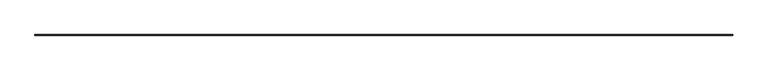
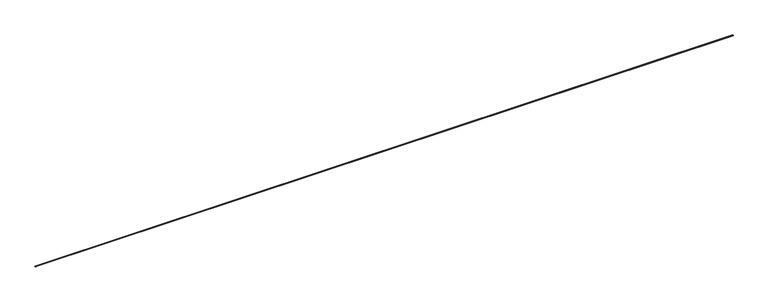
"""IFC4 building model written with IfcOpenShell, lengths in millimetres: proxy geometry, Inner panel:Inner panel:1:Inner panel:1 : Inner panel:Inner panel:300324:2:Inner panel:1:Inner panel:1 : Inner panel:Inner panel:300324:2 : Inner panel:Inner panel:1:Inner panel:1 : Inner panel:Inner panel:300324:300043:43 : Inner panel:Inner panel:1:Inner panel:1 : Inner panel:Inner panel:300324:2:Inner panel:1:Inner panel:1 : Inner panel:Inner panel:300324:2 : Inner panel:Inner panel:1:Inner panel:1 : Inner panel:Inner panel:300324:300043:308120."""

from ifc_helpers import new_model, si_unit, frame, origin, place, context, project, spatial, polyline, outline, extrude, source, transform, mapped, element, save


def generic_models_34035f40(model_context):
    return source(origin(), model_context, "Body", "SweptSolid", [
        extrude(outline(polyline([(-578217.5686142, 3944.3954083), (-578219.0886494, 3980.8762546), (-578261.9668057, 3979.0896648), (-578260.4467705, 3942.6088184), (-578277.1211775, 3941.9140515), (-578277.278418, 3945.6878244), (-578275.6895406, 3945.6878244), (-578275.6011422, 3943.5662637), (-578262.0989827, 3944.1288537), (-578263.619018, 3980.6097), (-578217.5686142, 3982.5284669), (-578216.0485789, 3946.0476205), (-578202.5464194, 3946.6102105), (-578202.6375715, 3948.7978597), (-578201.048694, 3948.7978597), (-578200.8942072, 3945.0901752), (-578217.5686142, 3944.3954083)])), frame((579104.5117239, 0.0, 0.0), z_axis=(1.0, 0.0, 0.0), x_axis=(0.0, 1.0, 0.0)), (0.0, 0.0, 1.0), 88442.8),
    ])


if __name__ == "__main__":
    model = new_model("IFC4")
    model_context = context("Model", 3, world=origin())
    ifc_project = project(units=[si_unit("LENGTHUNIT", "METRE", prefix="MILLI")], contexts=[model_context])
    site = spatial("IfcSite", under=ifc_project)
    building = spatial("IfcBuilding", under=site)
    placement = place(None, origin())
    generic_models_shape = generic_models_34035f40(model_context)
    element("IfcBuildingElementProxy", 1, Name="Inner panel:Inner panel:1:Inner panel:1 : Inner panel:Inner panel:300324:2:Inner panel:1:Inner panel:1 : Inner panel:Inner panel:300324:2 : Inner panel:Inner panel:1:Inner panel:1 : Inner panel:Inner panel:300324:300043:43 : Inner panel:Inner panel:1:Inner panel:1 : Inner panel:Inner panel:300324:2:Inner panel:1:Inner panel:1 : Inner panel:Inner panel:300324:2 : Inner panel:Inner panel:1:Inner panel:1 : Inner panel:Inner panel:300324:300043:308120", ObjectType="Inner panel:Inner panel:1:Inner panel:1 : Inner panel:Inner panel:300324:2:Inner panel:1:Inner panel:1 : Inner panel:Inner panel:300324:2 : Inner panel:Inner panel:1:Inner panel:1 : Inner panel:Inner panel:300324:300043:43 : Inner panel:Inner panel:1:Inner panel:1 : Inner panel:Inner panel:300324:2:Inner panel:1:Inner panel:1 : Inner panel:Inner panel:300324:2 : Inner panel:Inner panel:1:Inner panel:1 : Inner panel:Inner panel:300324:300043:308120", at=placement, inside=building, context=model_context, shape_type="MappedRepresentation", body=[
        mapped(generic_models_shape, transform((0.0, 0.0, 0.0), x_axis=(1.0, 0.0, 0.0), y_axis=(0.0, 1.0, 0.0), z_axis=(0.0, 0.0, 1.0))),
    ])
    save(model, "model.ifc")

# Revit data of these elements
# Type "Inner panel:Inner panel:1:Inner panel:1 : Inner panel:Inner panel:300324:2:Inner panel:1:Inner panel:1 : Inner panel:Inner panel:300324:2 : Inner panel:Inner panel:1:Inner panel:1 : Inner panel:Inner panel:300324:300043:43 : Inner panel:Inner panel:1:Inner panel:1 : Inner panel:Inner panel:300324:2:Inner panel:1:Inner panel:1 : Inner panel:Inner panel:300324:2 : Inner panel:Inner panel:1:Inner panel:1 : Inner panel:Inner panel:300324:300043:308120"
#   NameOverride = "Inner panel:Inner panel:1:Inner panel:1 : Inner panel:Inner panel:300324:2:Inner panel:1:Inner panel:1 : Inner panel:Inner panel:300324:2 : Inner panel:Inner panel:1:Inner panel:1 : Inner panel:Inner panel:300324:300043:308120"
#   ObjectTypeOverride = "Inner panel:1:Inner panel:1 : Inner panel:Inner panel:300324:2 : Inner panel:Inner panel:1:Inner panel:1 : Inner panel:Inner panel:300324:300043"
#   Reference = "Inner panel"
#   Tag = "308120"
# Element 1 (IfcBuildingElementProxy, "Inner panel:Inner panel:1:Inner panel:1 : Inner panel:Inner panel:300324:2:Inner panel:1:Inner panel:1 : Inner panel:Inner panel:300324:2 : Inner panel:Inner panel:1:Inner panel:1 : Inner panel:Inner panel:300324:300043:43 : Inner panel:Inner panel:1:Inner panel:1 : Inner panel:Inner panel:300324:2:Inner panel:1:Inner panel:1 : Inner panel:Inner panel:300324:2 : Inner panel:Inner panel:1:Inner panel:1 : Inner panel:Inner panel:300324:300043:308120")
#   Materials on its faces: "1 1/2\" HAT CHANNELS - SEE STRUCT. DWGs"
# Materials
#   "1 1/2\" HAT CHANNELS - SEE STRUCT. DWGs": class "Metal", colour RGB 189 187 185, transparency 0, Description = "Structural steel 50ksi", Cost = 0
